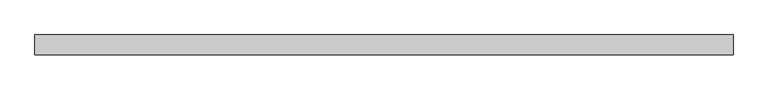
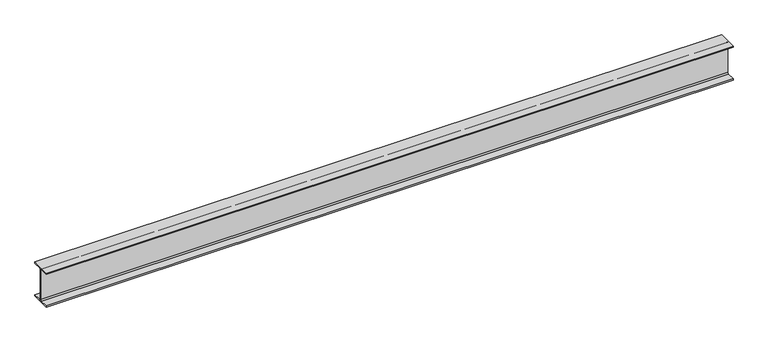
"""IFC4 building model written with IfcOpenShell, lengths in millimetres: beam geometry, Old_Steel Beam_H-KSD3502 : H_SB_ASB_H-350×175x7x11."""

from ifc_helpers import new_model, si_unit, point, frame, frame_2d, origin, place, context, project, spatial, polyline, circle_curve, trimmed, segment, composite_curve, outline, extrude, source, transform, mapped, element, save


def beam_7ac76af7(model_context):
    return source(origin(), model_context, "Body", "SweptSolid", [
        extrude(outline(composite_curve([segment(polyline([(82.5, -141.5), (82.5, -151.7), (-82.5, -151.7), (-82.5, -141.5), (-11.9, -141.5)]), True, "CONTINUOUS"), segment(trimmed(circle_curve(frame_2d((-11.9, -132.6)), 8.9), [point((-11.9, -141.5))], [point((-3.0, -132.6))], True, "CARTESIAN"), True, "CONTINUOUS"), segment(polyline([(-3.0, -132.6), (-3.0, 132.6)]), True, "CONTINUOUS"), segment(trimmed(circle_curve(frame_2d((-11.9, 132.6)), 8.9), [point((-3.0, 132.6))], [point((-11.9, 141.5))], True, "CARTESIAN"), True, "CONTINUOUS"), segment(polyline([(-11.9, 141.5), (-82.5, 141.5), (-82.5, 151.7), (82.5, 151.7), (82.5, 141.5), (11.9, 141.5)]), True, "CONTINUOUS"), segment(trimmed(circle_curve(frame_2d((11.9, 132.6)), 8.9), [point((11.9, 141.5))], [point((3.0, 132.6))], True, "CARTESIAN"), True, "CONTINUOUS"), segment(polyline([(3.0, 132.6), (3.0, -132.6)]), True, "CONTINUOUS"), segment(trimmed(circle_curve(frame_2d((11.9, -132.6)), 8.9), [point((3.0, -132.6))], [point((11.9, -141.5))], True, "CARTESIAN"), True, "CONTINUOUS"), segment(polyline([(11.9, -141.5), (82.5, -141.5)]), True, "CONTINUOUS")], self_intersect=False)), frame((-2920.1721181, 0.0, 0.0), z_axis=(1.0, 0.0, 0.0), x_axis=(0.0, 1.0, 0.0)), (0.0, 0.0, 1.0), 5810.1548079),
    ])


if __name__ == "__main__":
    model = new_model("IFC4")
    model_context = context("Model", 3, world=origin())
    ifc_project = project(units=[si_unit("LENGTHUNIT", "METRE", prefix="MILLI")], contexts=[model_context])
    site = spatial("IfcSite", under=ifc_project)
    building = spatial("IfcBuilding", under=site)
    placement = place(None, origin())
    beam_shape = beam_7ac76af7(model_context)
    element("IfcBeam", 1, ObjectType="Old_Steel Beam_H-KSD3502 : H_SB_ASB_H-350×175x7x11", at=placement, inside=building, context=model_context, shape_type="MappedRepresentation", body=[
        mapped(beam_shape, transform((0.0, 0.0, 0.0), x_axis=(1.0, 0.0, 0.0), y_axis=(0.0, 1.0, 0.0), z_axis=(0.0, 0.0, 1.0))),
    ])
    save(model, "model.ifc")

# Revit data of these elements
# Type "Old_Steel Beam_H-KSD3502 : H_SB_ASB_H-350×175x7x11"
#   Width = 17.5 cm
#   Web Thickness = 0.7 cm
#   Web Fillet = 1.4 cm
#   Warping Constant = 282290.0 cm⁶
#   Torsional Moment of Inertia = 19.4042 cm⁴
#   Torsional Modulus = 1.0 cm³
#   Section Area = 63.14 cm²
#   Plastic Modulus weak axis = 174.0 cm³
#   Plastic Modulus strong axis = 868.0 cm³
#   Perimeter = 1.36 m²/m
#   Nominal Weight = 49.60 kgf/m
#   Moment of Inertia weak axis = 984.00 cm⁴
#   Moment of Inertia strong axis = 13600.00 cm⁴
#   Height = 35.0 cm
#   Flange Thickness = 1.1 cm
#   Elastic Modulus weak axis = 112.0 cm³
#   Elastic Modulus strong axis = 775.0 cm³
#   Centroid Vertical = 17.5 cm
#   Centroid Horizontal = 8.75 cm
#   Length [instance default] = 1.5240 m
#   Structural Material [instance default] = Steel, 45-345
#   Assembly Code = ""
# Element 1 (IfcBeam, "Old_Steel Beam_H-KSD3502 : H_SB_ASB_H-350×175x7x11")
#   Structural Material = none
# Materials
#   "Steel, 45-345": class "Metal", colour RGB 189 187 185, transparency 0, Description = "Steel 345 MPa", Cost = 0
